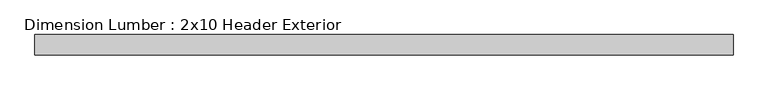
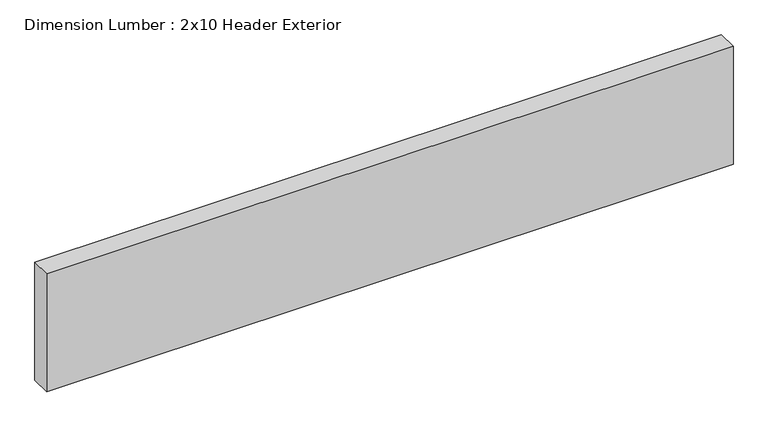
"""IFC4 building model written with IfcOpenShell, lengths in millimetres: beam geometry, Dimension Lumber : 2x10 Header Exterior."""

from ifc_helpers import new_model, si_unit, frame, origin, place, context, project, spatial, polyline, outline, extrude, source, transform, mapped, element, save


def dimension_lumber_2x10_header_exterior_8d927054(model_context):
    return source(origin(), model_context, "Body", "SweptSolid", [
        extrude(outline(polyline([(468.709375, 19.05), (468.709375, -19.05), (-826.690625, -19.05), (-826.690625, 19.05), (468.709375, 19.05)])), frame((0.0, 0.0, -117.475), z_axis=(0.0, 0.0, 1.0), x_axis=(1.0, 0.0, 0.0)), (0.0, 0.0, 1.0), 234.95),
    ])


if __name__ == "__main__":
    model = new_model("IFC4")
    model_context = context("Model", 3, world=origin())
    ifc_project = project(units=[si_unit("LENGTHUNIT", "METRE", prefix="MILLI")], contexts=[model_context])
    site = spatial("IfcSite", under=ifc_project)
    building = spatial("IfcBuilding", under=site)
    placement = place(None, origin())
    dimension_lumber_2x10_header_exterior_shape = dimension_lumber_2x10_header_exterior_8d927054(model_context)
    element("IfcBeam", 1, ObjectType="Dimension Lumber : 2x10 Header Exterior", at=placement, inside=building, context=model_context, shape_type="MappedRepresentation", body=[
        mapped(dimension_lumber_2x10_header_exterior_shape, transform((0.0, 0.0, 0.0), x_axis=(1.0, 0.0, 0.0), y_axis=(0.0, 1.0, 0.0), z_axis=(0.0, 0.0, 1.0))),
    ])
    save(model, "model.ifc")

# Revit data of these elements
# Type "Dimension Lumber : 2x10 Header Exterior"
#   Assembly Code = "B10"
#   A = 0.0963889 SF
#   Length [instance default] = 5' - 0"
#   b = 0' - 1 1/2"
#   d = 0' - 9 1/4"
#   Structural Material [instance default] = Softwood, Lumber
# Element 1 (IfcBeam, "Dimension Lumber : 2x10 Header Exterior")
#   Structural Material = Douglas Fir #2
#   Materials on its faces: "Douglas Fir #2"
# Materials
#   "Softwood, Lumber": class "Wood", colour RGB 223 192 134, transparency 0, Description = "Pinus Echinata", Cost = 0
#   "Douglas Fir #2": class "Wood", colour RGB 223 192 134, transparency 0, Description = "Pinus Echinata", Cost = 0
